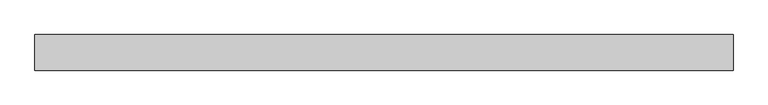
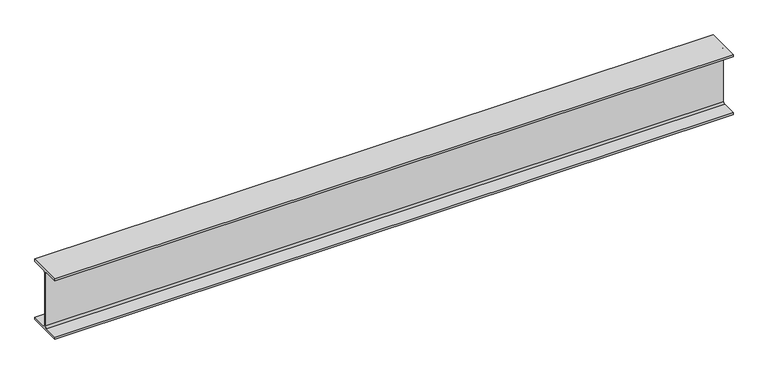
"""IFC4 building model written with IfcOpenShell, lengths in millimetres: beam geometry, Steel Beam_H-KSD3502 : H_SB_ASB_H-200x200x8x12."""

import ifcopenshell
import ifcopenshell.guid

model = None  # the IFC model being written
_history = None  # IfcOwnerHistory: only IFC2X3 demands one
_inside = {}  # id of a spatial element -> (the spatial element, [elements in it])
_under = {}  # id of a project, library or spatial element -> (it, [spatial elements below it])
_declared = {}  # id of a project -> (the project, [libraries it declares])
_typed = {}  # id of a type object -> (the type object, [elements of that type])
_made_of = {}  # id of a material, layer set ... -> (it, [elements and type objects made of it])


def new_model(schema):
    """Start an empty IFC model of exactly this schema.

    Asked for "IFC4X3", IfcOpenShell would pick the latest addendum, in which some entities
    have other attributes; the version numbers below select the first issue.
    IFC2X3 requires an IfcOwnerHistory on every rooted entity: one is made here for all.
    """
    global model, _history
    if schema == "IFC4X3":
        model = ifcopenshell.file(schema_version=(4, 3, 0, 0))
    else:
        model = ifcopenshell.file(schema=schema)
    _inside.clear()
    _under.clear()
    _declared.clear()
    _typed.clear()
    _made_of.clear()
    _history = None
    if model.schema == "IFC2X3":
        org = make("IfcOrganization", Name="unknown")
        user = make(
            "IfcPersonAndOrganization",
            ThePerson=make("IfcPerson", FamilyName="unknown"),
            TheOrganization=org,
        )
        app = make(
            "IfcApplication",
            ApplicationDeveloper=org,
            Version="unknown",
            ApplicationFullName="unknown",
            ApplicationIdentifier="unknown",
        )
        _history = make(
            "IfcOwnerHistory",
            OwningUser=user,
            OwningApplication=app,
            ChangeAction="ADDED",
            CreationDate=0,
        )
    return model


def make(cls, **values):
    """One entity of the class cls with the attributes given. An attribute that is None is left unset."""
    return model.create_entity(
        cls, **{name: value for name, value in values.items() if value is not None}
    )


def rooted(cls, **values):
    """An entity with a GlobalId (a new one), such as an element, a storey or a relation."""
    return make(cls, GlobalId=ifcopenshell.guid.new(), OwnerHistory=_history, **values)


def si_unit(unit_type, name, prefix=None):
    """IfcSIUnit, for example si_unit("LENGTHUNIT", "METRE", prefix="MILLI")."""
    return make("IfcSIUnit", UnitType=unit_type, Prefix=prefix, Name=name)


def assignment(units):
    """IfcUnitAssignment: the units of a project."""
    return None if units is None else make("IfcUnitAssignment", Units=units)


def point(xyz):
    """IfcCartesianPoint."""
    return None if xyz is None else make("IfcCartesianPoint", Coordinates=xyz)


def direction(xyz):
    """IfcDirection."""
    return None if xyz is None else make("IfcDirection", DirectionRatios=xyz)


def frame(location, z_axis=None, x_axis=None):
    """IfcAxis2Placement3D, a coordinate frame: its origin and axes. An axis left out is left unset."""
    return make(
        "IfcAxis2Placement3D",
        Location=point(location),
        Axis=direction(z_axis),
        RefDirection=direction(x_axis),
    )


def frame_2d(location, x_axis=None):
    """IfcAxis2Placement2D, a coordinate frame in the plane: its origin and x axis."""
    return make(
        "IfcAxis2Placement2D", Location=point(location), RefDirection=direction(x_axis)
    )


def origin():
    """The frame at (0, 0, 0) with its axes left unset."""
    return frame((0.0, 0.0, 0.0))


def place(relative_to, where):
    """IfcLocalPlacement: puts the frame where relative to a parent placement (None: the world)."""
    return make(
        "IfcLocalPlacement", PlacementRelTo=relative_to, RelativePlacement=where
    )


def context(
    kind, dimensions, precision=None, world=None, true_north=None, identifier=None
):
    """IfcGeometricRepresentationContext, for example the 3D "Model" context."""
    return make(
        "IfcGeometricRepresentationContext",
        ContextIdentifier=identifier,
        ContextType=kind,
        CoordinateSpaceDimension=dimensions,
        Precision=precision,
        WorldCoordinateSystem=world,
        TrueNorth=true_north,
    )


def project(units=None, contexts=None):
    """IfcProject with its units and contexts."""
    return rooted(
        "IfcProject",
        Name="project",
        RepresentationContexts=contexts,
        UnitsInContext=assignment(units),
    )


def spatial(cls, under=None, at=None, **own):
    """A site, building, storey or space (cls), placed at a placement, below another one or the project."""
    s = rooted(cls, ObjectPlacement=at, **own)
    if under is not None:
        _under.setdefault(under.id(), (under, []))[1].append(s)
    return s


def polyline(points):
    """IfcPolyline through the points."""
    return make("IfcPolyline", Points=[point(p) for p in points])


def circle_curve(where, radius):
    """IfcCircle in the frame where."""
    return make("IfcCircle", Position=where, Radius=radius)


def trimmed(basis, trim1, trim2, sense, master):
    """IfcTrimmedCurve: the piece of a basis curve between two trims."""
    return make(
        "IfcTrimmedCurve",
        BasisCurve=basis,
        Trim1=trim1,
        Trim2=trim2,
        SenseAgreement=sense,
        MasterRepresentation=master,
    )


def segment(curve, same_sense, transition):
    """IfcCompositeCurveSegment."""
    return make(
        "IfcCompositeCurveSegment",
        Transition=transition,
        SameSense=same_sense,
        ParentCurve=curve,
    )


def composite_curve(segments, self_intersect=None):
    """IfcCompositeCurve: segments joined end to end."""
    return make("IfcCompositeCurve", Segments=segments, SelfIntersect=self_intersect)


def outline(outer, holes=None, kind="AREA"):
    """IfcArbitraryClosedProfileDef: a profile drawn as a closed curve; with holes, ...WithVoids."""
    if holes is None:
        return make("IfcArbitraryClosedProfileDef", ProfileType=kind, OuterCurve=outer)
    return make(
        "IfcArbitraryProfileDefWithVoids",
        ProfileType=kind,
        OuterCurve=outer,
        InnerCurves=holes,
    )


def extrude(swept, where, along, depth):
    """IfcExtrudedAreaSolid: the profile swept, set in the frame where, extruded along a direction by depth."""
    return make(
        "IfcExtrudedAreaSolid",
        SweptArea=swept,
        Position=where,
        ExtrudedDirection=direction(along),
        Depth=depth,
    )


def shape(context_of_items, identifier, shape_type, items):
    """IfcShapeRepresentation: the items that make up one representation, for example the "Body"."""
    return make(
        "IfcShapeRepresentation",
        ContextOfItems=context_of_items,
        RepresentationIdentifier=identifier,
        RepresentationType=shape_type,
        Items=items,
    )


def source(mapping_origin, context_of_items, identifier, shape_type, items):
    """IfcRepresentationMap: a shape defined once, which mapped items show again and again."""
    return make(
        "IfcRepresentationMap",
        MappingOrigin=mapping_origin,
        MappedRepresentation=shape(context_of_items, identifier, shape_type, items),
    )


def transform(
    local_origin,
    x_axis=None,
    y_axis=None,
    z_axis=None,
    scale=None,
    scale2=None,
    scale3=None,
    uniform=True,
):
    """IfcCartesianTransformationOperator3D, or its non-uniform kind. x_axis, y_axis, z_axis: its Axis1, 2, 3."""
    if uniform:
        return make(
            "IfcCartesianTransformationOperator3D",
            Axis1=direction(x_axis),
            Axis2=direction(y_axis),
            LocalOrigin=point(local_origin),
            Scale=scale,
            Axis3=direction(z_axis),
        )
    return make(
        "IfcCartesianTransformationOperator3DnonUniform",
        Axis1=direction(x_axis),
        Axis2=direction(y_axis),
        LocalOrigin=point(local_origin),
        Scale=scale,
        Axis3=direction(z_axis),
        Scale2=scale2,
        Scale3=scale3,
    )


def mapped(mapping_source, mapping_target):
    """IfcMappedItem: shows the shape of a source again, moved by a transform."""
    return make(
        "IfcMappedItem", MappingSource=mapping_source, MappingTarget=mapping_target
    )


def made_of(thing, what):
    """Note that an element or type object is made of a material, layer set ...; save() writes the relation."""
    if what is not None:
        _made_of.setdefault(what.id(), (what, []))[1].append(thing)
    return thing


def element(
    cls,
    number,
    at=None,
    inside=None,
    cuts=None,
    type_object=None,
    material=None,
    context=None,
    identifier="Body",
    shape_type=None,
    held_by="IfcProductDefinitionShape",
    body=None,
    shapes=None,
    **own,
):
    """One element of the class cls, such as IfcWall. Its Tag is "e" and its number.

    at: its placement. inside: the storey or other place that contains it. cuts: it is an
    opening in that element (IfcRelVoidsElement). A single representation is given by context,
    identifier, shape_type and body (its items); several are given by shapes. held_by: the class
    of the entity that holds the representations. save() writes the other relations.
    """
    e = rooted(cls, Tag="e%d" % number, ObjectPlacement=at, **own)
    if body is not None:
        shapes = [shape(context, identifier, shape_type, body)]
    if shapes is not None:
        e.Representation = make(held_by, Representations=shapes)
    if inside is not None:
        _inside.setdefault(inside.id(), (inside, []))[1].append(e)
    if cuts is not None:
        rooted(
            "IfcRelVoidsElement", RelatingBuildingElement=cuts, RelatedOpeningElement=e
        )
    if type_object is not None:
        _typed.setdefault(type_object.id(), (type_object, []))[1].append(e)
    return made_of(e, material)


def aggregate(whole, parts):
    """IfcRelAggregates: a whole, such as a stair, and the parts it consists of."""
    return rooted("IfcRelAggregates", RelatingObject=whole, RelatedObjects=parts)


def save(model, path):
    """Write the relations noted so far, then the file.

    IfcRelAggregates (storeys below a building ...), IfcRelContainedInSpatialStructure (elements
    in a storey), IfcRelDefinesByType, IfcRelAssociatesMaterial and IfcRelDeclares: one each for
    every whole, place, type object, material and project.
    """
    for whole, parts in _under.values():
        aggregate(whole, parts)
    for where, things in _inside.values():
        rooted(
            "IfcRelContainedInSpatialStructure",
            RelatedElements=things,
            RelatingStructure=where,
        )
    for kind, things in _typed.values():
        rooted("IfcRelDefinesByType", RelatedObjects=things, RelatingType=kind)
    for what, things in _made_of.values():
        rooted("IfcRelAssociatesMaterial", RelatedObjects=things, RelatingMaterial=what)
    for by, libraries in _declared.values():
        rooted("IfcRelDeclares", RelatingContext=by, RelatedDefinitions=libraries)
    model.write(path)


def beam_e6466eaf(model_context):
    return source(origin(), model_context, "Body", "SweptSolid", [
        extrude(outline(composite_curve([segment(polyline([(82.5, -141.5), (82.5, -151.7), (-82.5, -151.7), (-82.5, -141.5), (-11.9, -141.5)]), True, "CONTINUOUS"), segment(trimmed(circle_curve(frame_2d((-11.9, -132.6)), 8.9), [point((-11.9, -141.5))], [point((-3.0, -132.6))], True, "CARTESIAN"), True, "CONTINUOUS"), segment(polyline([(-3.0, -132.6), (-3.0, 132.6)]), True, "CONTINUOUS"), segment(trimmed(circle_curve(frame_2d((-11.9, 132.6)), 8.9), [point((-3.0, 132.6))], [point((-11.9, 141.5))], True, "CARTESIAN"), True, "CONTINUOUS"), segment(polyline([(-11.9, 141.5), (-82.5, 141.5), (-82.5, 151.7), (82.5, 151.7), (82.5, 141.5), (11.9, 141.5)]), True, "CONTINUOUS"), segment(trimmed(circle_curve(frame_2d((11.9, 132.6)), 8.9), [point((11.9, 141.5))], [point((3.0, 132.6))], True, "CARTESIAN"), True, "CONTINUOUS"), segment(polyline([(3.0, 132.6), (3.0, -132.6)]), True, "CONTINUOUS"), segment(trimmed(circle_curve(frame_2d((11.9, -132.6)), 8.9), [point((3.0, -132.6))], [point((11.9, -141.5))], True, "CARTESIAN"), True, "CONTINUOUS"), segment(polyline([(11.9, -141.5), (82.5, -141.5)]), True, "CONTINUOUS")], self_intersect=False)), frame((-1409.9859537, 0.0, 0.0), z_axis=(1.0, 0.0, 0.0), x_axis=(0.0, 1.0, 0.0)), (0.0, 0.0, 1.0), 3231.4633723),
    ])


if __name__ == "__main__":
    model = new_model("IFC4")
    model_context = context("Model", 3, world=origin())
    ifc_project = project(units=[si_unit("LENGTHUNIT", "METRE", prefix="MILLI")], contexts=[model_context])
    site = spatial("IfcSite", under=ifc_project)
    building = spatial("IfcBuilding", under=site)
    placement = place(None, origin())
    beam_shape = beam_e6466eaf(model_context)
    element("IfcBeam", 1, ObjectType="Steel Beam_H-KSD3502 : H_SB_ASB_H-200x200x8x12", at=placement, inside=building, context=model_context, shape_type="MappedRepresentation", body=[
        mapped(beam_shape, transform((0.0, 0.0, 0.0), x_axis=(1.0, 0.0, 0.0), y_axis=(0.0, 1.0, 0.0), z_axis=(0.0, 0.0, 1.0))),
    ])
    save(model, "model.ifc")

# Revit data of these elements
# Type "Steel Beam_H-KSD3502 : H_SB_ASB_H-200x200x8x12"
#   Width = 20.0 cm
#   Web Thickness = 0.8 cm
#   Web Fillet = 1.3 cm
#   Warping Constant = 141376.0 cm⁶
#   Torsional Moment of Inertia = 26.2485 cm⁴
#   Torsional Modulus = 1.0 cm³
#   Section Area = 63.53 cm²
#   Plastic Modulus weak axis = 244.0 cm³
#   Plastic Modulus strong axis = 525.0 cm³
#   Perimeter = 1.16 m²/m
#   Nominal Weight = 49.90 kgf/m
#   Moment of Inertia weak axis = 1600.00 cm⁴
#   Moment of Inertia strong axis = 4720.00 cm⁴
#   Height = 20.0 cm
#   Flange Thickness = 1.2 cm
#   Elastic Modulus weak axis = 160.0 cm³
#   Elastic Modulus strong axis = 472.0 cm³
#   Centroid Vertical = 10.0 cm
#   Centroid Horizontal = 10.0 cm
#   Length [instance default] = 1.5240 m
#   Structural Material [instance default] = Steel, 45-345
#   Assembly Code = ""
# Element 1 (IfcBeam, "Steel Beam_H-KSD3502 : H_SB_ASB_H-200x200x8x12")
#   Structural Material = none
# Materials
#   "Steel, 45-345": class "Metal", colour RGB 189 187 185, transparency 0, Description = "Steel 345 MPa", Cost = 0
